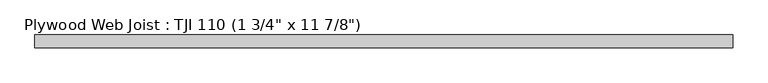
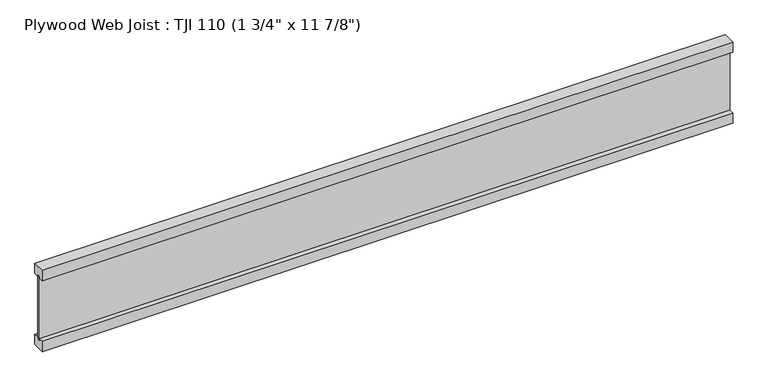
"""IFC4 building model written with IfcOpenShell, lengths in millimetres: beam geometry."""

import ifcopenshell
import ifcopenshell.guid

model = None  # the IFC model being written
_history = None  # IfcOwnerHistory: only IFC2X3 demands one
_inside = {}  # id of a spatial element -> (the spatial element, [elements in it])
_under = {}  # id of a project, library or spatial element -> (it, [spatial elements below it])
_declared = {}  # id of a project -> (the project, [libraries it declares])
_typed = {}  # id of a type object -> (the type object, [elements of that type])
_made_of = {}  # id of a material, layer set ... -> (it, [elements and type objects made of it])


def new_model(schema):
    """Start an empty IFC model of exactly this schema.

    Asked for "IFC4X3", IfcOpenShell would pick the latest addendum, in which some entities
    have other attributes; the version numbers below select the first issue.
    IFC2X3 requires an IfcOwnerHistory on every rooted entity: one is made here for all.
    """
    global model, _history
    if schema == "IFC4X3":
        model = ifcopenshell.file(schema_version=(4, 3, 0, 0))
    else:
        model = ifcopenshell.file(schema=schema)
    _inside.clear()
    _under.clear()
    _declared.clear()
    _typed.clear()
    _made_of.clear()
    _history = None
    if model.schema == "IFC2X3":
        org = make("IfcOrganization", Name="unknown")
        user = make(
            "IfcPersonAndOrganization",
            ThePerson=make("IfcPerson", FamilyName="unknown"),
            TheOrganization=org,
        )
        app = make(
            "IfcApplication",
            ApplicationDeveloper=org,
            Version="unknown",
            ApplicationFullName="unknown",
            ApplicationIdentifier="unknown",
        )
        _history = make(
            "IfcOwnerHistory",
            OwningUser=user,
            OwningApplication=app,
            ChangeAction="ADDED",
            CreationDate=0,
        )
    return model


def make(cls, **values):
    """One entity of the class cls with the attributes given. An attribute that is None is left unset."""
    return model.create_entity(
        cls, **{name: value for name, value in values.items() if value is not None}
    )


def rooted(cls, **values):
    """An entity with a GlobalId (a new one), such as an element, a storey or a relation."""
    return make(cls, GlobalId=ifcopenshell.guid.new(), OwnerHistory=_history, **values)


def si_unit(unit_type, name, prefix=None):
    """IfcSIUnit, for example si_unit("LENGTHUNIT", "METRE", prefix="MILLI")."""
    return make("IfcSIUnit", UnitType=unit_type, Prefix=prefix, Name=name)


def assignment(units):
    """IfcUnitAssignment: the units of a project."""
    return None if units is None else make("IfcUnitAssignment", Units=units)


def point(xyz):
    """IfcCartesianPoint."""
    return None if xyz is None else make("IfcCartesianPoint", Coordinates=xyz)


def direction(xyz):
    """IfcDirection."""
    return None if xyz is None else make("IfcDirection", DirectionRatios=xyz)


def frame(location, z_axis=None, x_axis=None):
    """IfcAxis2Placement3D, a coordinate frame: its origin and axes. An axis left out is left unset."""
    return make(
        "IfcAxis2Placement3D",
        Location=point(location),
        Axis=direction(z_axis),
        RefDirection=direction(x_axis),
    )


def origin():
    """The frame at (0, 0, 0) with its axes left unset."""
    return frame((0.0, 0.0, 0.0))


def place(relative_to, where):
    """IfcLocalPlacement: puts the frame where relative to a parent placement (None: the world)."""
    return make(
        "IfcLocalPlacement", PlacementRelTo=relative_to, RelativePlacement=where
    )


def context(
    kind, dimensions, precision=None, world=None, true_north=None, identifier=None
):
    """IfcGeometricRepresentationContext, for example the 3D "Model" context."""
    return make(
        "IfcGeometricRepresentationContext",
        ContextIdentifier=identifier,
        ContextType=kind,
        CoordinateSpaceDimension=dimensions,
        Precision=precision,
        WorldCoordinateSystem=world,
        TrueNorth=true_north,
    )


def project(units=None, contexts=None):
    """IfcProject with its units and contexts."""
    return rooted(
        "IfcProject",
        Name="project",
        RepresentationContexts=contexts,
        UnitsInContext=assignment(units),
    )


def spatial(cls, under=None, at=None, **own):
    """A site, building, storey or space (cls), placed at a placement, below another one or the project."""
    s = rooted(cls, ObjectPlacement=at, **own)
    if under is not None:
        _under.setdefault(under.id(), (under, []))[1].append(s)
    return s


def polyline(points):
    """IfcPolyline through the points."""
    return make("IfcPolyline", Points=[point(p) for p in points])


def outline(outer, holes=None, kind="AREA"):
    """IfcArbitraryClosedProfileDef: a profile drawn as a closed curve; with holes, ...WithVoids."""
    if holes is None:
        return make("IfcArbitraryClosedProfileDef", ProfileType=kind, OuterCurve=outer)
    return make(
        "IfcArbitraryProfileDefWithVoids",
        ProfileType=kind,
        OuterCurve=outer,
        InnerCurves=holes,
    )


def extrude(swept, where, along, depth):
    """IfcExtrudedAreaSolid: the profile swept, set in the frame where, extruded along a direction by depth."""
    return make(
        "IfcExtrudedAreaSolid",
        SweptArea=swept,
        Position=where,
        ExtrudedDirection=direction(along),
        Depth=depth,
    )


def shape(context_of_items, identifier, shape_type, items):
    """IfcShapeRepresentation: the items that make up one representation, for example the "Body"."""
    return make(
        "IfcShapeRepresentation",
        ContextOfItems=context_of_items,
        RepresentationIdentifier=identifier,
        RepresentationType=shape_type,
        Items=items,
    )


def source(mapping_origin, context_of_items, identifier, shape_type, items):
    """IfcRepresentationMap: a shape defined once, which mapped items show again and again."""
    return make(
        "IfcRepresentationMap",
        MappingOrigin=mapping_origin,
        MappedRepresentation=shape(context_of_items, identifier, shape_type, items),
    )


def transform(
    local_origin,
    x_axis=None,
    y_axis=None,
    z_axis=None,
    scale=None,
    scale2=None,
    scale3=None,
    uniform=True,
):
    """IfcCartesianTransformationOperator3D, or its non-uniform kind. x_axis, y_axis, z_axis: its Axis1, 2, 3."""
    if uniform:
        return make(
            "IfcCartesianTransformationOperator3D",
            Axis1=direction(x_axis),
            Axis2=direction(y_axis),
            LocalOrigin=point(local_origin),
            Scale=scale,
            Axis3=direction(z_axis),
        )
    return make(
        "IfcCartesianTransformationOperator3DnonUniform",
        Axis1=direction(x_axis),
        Axis2=direction(y_axis),
        LocalOrigin=point(local_origin),
        Scale=scale,
        Axis3=direction(z_axis),
        Scale2=scale2,
        Scale3=scale3,
    )


def mapped(mapping_source, mapping_target):
    """IfcMappedItem: shows the shape of a source again, moved by a transform."""
    return make(
        "IfcMappedItem", MappingSource=mapping_source, MappingTarget=mapping_target
    )


def made_of(thing, what):
    """Note that an element or type object is made of a material, layer set ...; save() writes the relation."""
    if what is not None:
        _made_of.setdefault(what.id(), (what, []))[1].append(thing)
    return thing


def element(
    cls,
    number,
    at=None,
    inside=None,
    cuts=None,
    type_object=None,
    material=None,
    context=None,
    identifier="Body",
    shape_type=None,
    held_by="IfcProductDefinitionShape",
    body=None,
    shapes=None,
    **own,
):
    """One element of the class cls, such as IfcWall. Its Tag is "e" and its number.

    at: its placement. inside: the storey or other place that contains it. cuts: it is an
    opening in that element (IfcRelVoidsElement). A single representation is given by context,
    identifier, shape_type and body (its items); several are given by shapes. held_by: the class
    of the entity that holds the representations. save() writes the other relations.
    """
    e = rooted(cls, Tag="e%d" % number, ObjectPlacement=at, **own)
    if body is not None:
        shapes = [shape(context, identifier, shape_type, body)]
    if shapes is not None:
        e.Representation = make(held_by, Representations=shapes)
    if inside is not None:
        _inside.setdefault(inside.id(), (inside, []))[1].append(e)
    if cuts is not None:
        rooted(
            "IfcRelVoidsElement", RelatingBuildingElement=cuts, RelatedOpeningElement=e
        )
    if type_object is not None:
        _typed.setdefault(type_object.id(), (type_object, []))[1].append(e)
    return made_of(e, material)


def aggregate(whole, parts):
    """IfcRelAggregates: a whole, such as a stair, and the parts it consists of."""
    return rooted("IfcRelAggregates", RelatingObject=whole, RelatedObjects=parts)


def save(model, path):
    """Write the relations noted so far, then the file.

    IfcRelAggregates (storeys below a building ...), IfcRelContainedInSpatialStructure (elements
    in a storey), IfcRelDefinesByType, IfcRelAssociatesMaterial and IfcRelDeclares: one each for
    every whole, place, type object, material and project.
    """
    for whole, parts in _under.values():
        aggregate(whole, parts)
    for where, things in _inside.values():
        rooted(
            "IfcRelContainedInSpatialStructure",
            RelatedElements=things,
            RelatingStructure=where,
        )
    for kind, things in _typed.values():
        rooted("IfcRelDefinesByType", RelatedObjects=things, RelatingType=kind)
    for what, things in _made_of.values():
        rooted("IfcRelAssociatesMaterial", RelatedObjects=things, RelatingMaterial=what)
    for by, libraries in _declared.values():
        rooted("IfcRelDeclares", RelatingContext=by, RelatedDefinitions=libraries)
    model.write(path)


def beam_4fc2050d(model_context):
    return source(origin(), model_context, "Body", "SweptSolid", [
        extrude(outline(polyline([(-22.225, 150.8125), (22.225, 150.8125), (22.225, 112.7125), (4.7625, 112.7125), (4.7625, 119.0625), (-4.7625, 119.0625), (-4.7625, 112.7125), (-22.225, 112.7125), (-22.225, 150.8125)])), frame((-1200.15, 0.0, 0.0), z_axis=(1.0, 0.0, 0.0), x_axis=(0.0, 1.0, 0.0)), (0.0, 0.0, 1.0), 2428.875),
        extrude(outline(polyline([(22.225, -112.7125), (22.225, -150.8125), (-22.225, -150.8125), (-22.225, -112.7125), (-4.7625, -112.7125), (-4.7625, -118.3285374), (4.7625, -118.3285374), (4.7625, -112.7125), (22.225, -112.7125)])), frame((-1200.15, 0.0, 0.0), z_axis=(1.0, 0.0, 0.0), x_axis=(0.0, 1.0, 0.0)), (0.0, 0.0, 1.0), 2428.875),
        extrude(outline(polyline([(1228.725, 4.7625), (1228.725, -4.7625), (-1200.15, -4.7625), (-1200.15, 4.7625), (1228.725, 4.7625)])), frame((0.0, 0.0, -118.3285374), z_axis=(0.0, 0.0, 1.0), x_axis=(1.0, 0.0, 0.0)), (0.0, 0.0, 1.0), 237.3910374),
    ])


if __name__ == "__main__":
    model = new_model("IFC4")
    model_context = context("Model", 3, world=origin())
    ifc_project = project(units=[si_unit("LENGTHUNIT", "METRE", prefix="MILLI")], contexts=[model_context])
    site = spatial("IfcSite", under=ifc_project)
    building = spatial("IfcBuilding", under=site)
    placement = place(None, origin())
    beam_shape = beam_4fc2050d(model_context)
    element("IfcBeam", 1, ObjectType="Plywood Web Joist : TJI 110 (1 3/4\" x 11 7/8\")", at=placement, inside=building, context=model_context, shape_type="MappedRepresentation", body=[
        mapped(beam_shape, transform((0.0, 0.0, 0.0), x_axis=(1.0, 0.0, 0.0), y_axis=(0.0, 1.0, 0.0), z_axis=(0.0, 0.0, 1.0))),
    ])
    save(model, "model.ifc")

# Revit data of these elements
# Type "Plywood Web Joist : TJI 110 (1 3/4\" x 11 7/8\")"
#   Assembly Code = "B10"
#   Length [instance default] = 5' - 0"
#   b = 0' - 1 3/4"
#   d = 0' - 11 7/8"
#   Structural Material [instance default] = Softwood, Lumber
# Element 1 (IfcBeam, "Plywood Web Joist : TJI 110 (1 3/4\" x 11 7/8\")")
#   Materials on its faces: "Softwood, Lumber"
# Materials
#   "Softwood, Lumber": class "Wood", colour RGB 144 113 62, transparency 0, Description = "Pinus Echinata", Cost = 0
